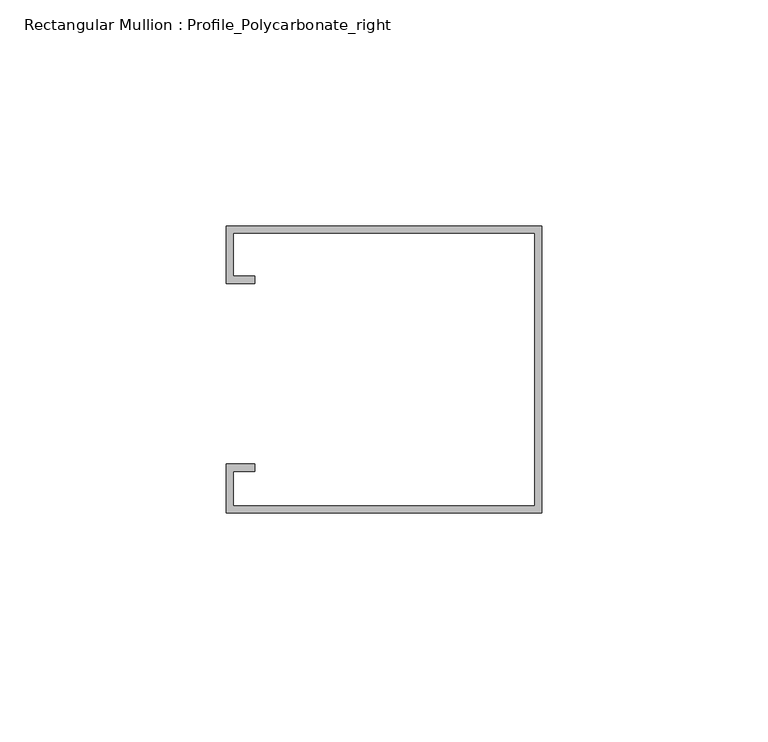
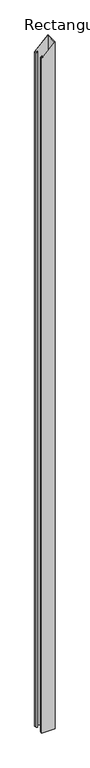
"""IFC4 building model written with IfcOpenShell, lengths in millimetres: member geometry, Rectangular Mullion : Profile_Polycarbonate_right."""

import ifcopenshell
import ifcopenshell.guid

model = None  # the IFC model being written
_history = None  # IfcOwnerHistory: only IFC2X3 demands one
_inside = {}  # id of a spatial element -> (the spatial element, [elements in it])
_under = {}  # id of a project, library or spatial element -> (it, [spatial elements below it])
_declared = {}  # id of a project -> (the project, [libraries it declares])
_typed = {}  # id of a type object -> (the type object, [elements of that type])
_made_of = {}  # id of a material, layer set ... -> (it, [elements and type objects made of it])


def new_model(schema):
    """Start an empty IFC model of exactly this schema.

    Asked for "IFC4X3", IfcOpenShell would pick the latest addendum, in which some entities
    have other attributes; the version numbers below select the first issue.
    IFC2X3 requires an IfcOwnerHistory on every rooted entity: one is made here for all.
    """
    global model, _history
    if schema == "IFC4X3":
        model = ifcopenshell.file(schema_version=(4, 3, 0, 0))
    else:
        model = ifcopenshell.file(schema=schema)
    _inside.clear()
    _under.clear()
    _declared.clear()
    _typed.clear()
    _made_of.clear()
    _history = None
    if model.schema == "IFC2X3":
        org = make("IfcOrganization", Name="unknown")
        user = make(
            "IfcPersonAndOrganization",
            ThePerson=make("IfcPerson", FamilyName="unknown"),
            TheOrganization=org,
        )
        app = make(
            "IfcApplication",
            ApplicationDeveloper=org,
            Version="unknown",
            ApplicationFullName="unknown",
            ApplicationIdentifier="unknown",
        )
        _history = make(
            "IfcOwnerHistory",
            OwningUser=user,
            OwningApplication=app,
            ChangeAction="ADDED",
            CreationDate=0,
        )
    return model


def make(cls, **values):
    """One entity of the class cls with the attributes given. An attribute that is None is left unset."""
    return model.create_entity(
        cls, **{name: value for name, value in values.items() if value is not None}
    )


def rooted(cls, **values):
    """An entity with a GlobalId (a new one), such as an element, a storey or a relation."""
    return make(cls, GlobalId=ifcopenshell.guid.new(), OwnerHistory=_history, **values)


def si_unit(unit_type, name, prefix=None):
    """IfcSIUnit, for example si_unit("LENGTHUNIT", "METRE", prefix="MILLI")."""
    return make("IfcSIUnit", UnitType=unit_type, Prefix=prefix, Name=name)


def assignment(units):
    """IfcUnitAssignment: the units of a project."""
    return None if units is None else make("IfcUnitAssignment", Units=units)


def point(xyz):
    """IfcCartesianPoint."""
    return None if xyz is None else make("IfcCartesianPoint", Coordinates=xyz)


def direction(xyz):
    """IfcDirection."""
    return None if xyz is None else make("IfcDirection", DirectionRatios=xyz)


def frame(location, z_axis=None, x_axis=None):
    """IfcAxis2Placement3D, a coordinate frame: its origin and axes. An axis left out is left unset."""
    return make(
        "IfcAxis2Placement3D",
        Location=point(location),
        Axis=direction(z_axis),
        RefDirection=direction(x_axis),
    )


def origin():
    """The frame at (0, 0, 0) with its axes left unset."""
    return frame((0.0, 0.0, 0.0))


def place(relative_to, where):
    """IfcLocalPlacement: puts the frame where relative to a parent placement (None: the world)."""
    return make(
        "IfcLocalPlacement", PlacementRelTo=relative_to, RelativePlacement=where
    )


def context(
    kind, dimensions, precision=None, world=None, true_north=None, identifier=None
):
    """IfcGeometricRepresentationContext, for example the 3D "Model" context."""
    return make(
        "IfcGeometricRepresentationContext",
        ContextIdentifier=identifier,
        ContextType=kind,
        CoordinateSpaceDimension=dimensions,
        Precision=precision,
        WorldCoordinateSystem=world,
        TrueNorth=true_north,
    )


def project(units=None, contexts=None):
    """IfcProject with its units and contexts."""
    return rooted(
        "IfcProject",
        Name="project",
        RepresentationContexts=contexts,
        UnitsInContext=assignment(units),
    )


def spatial(cls, under=None, at=None, **own):
    """A site, building, storey or space (cls), placed at a placement, below another one or the project."""
    s = rooted(cls, ObjectPlacement=at, **own)
    if under is not None:
        _under.setdefault(under.id(), (under, []))[1].append(s)
    return s


def faces_of(points, faces, orient=None, outer=None):
    """IfcFace entities. A face is a list of loops; a loop is a list of indices into points, from 0.

    orient and outer hold one flag for each loop. By default every Orientation is true, the
    first loop of a face is its IfcFaceOuterBound and the others are IfcFaceBound.
    """
    made = []
    for i, loops in enumerate(faces):
        bounds = []
        for j, loop in enumerate(loops):
            is_outer = j == 0 if outer is None else outer[i][j]
            bounds.append(
                make(
                    "IfcFaceOuterBound" if is_outer else "IfcFaceBound",
                    Bound=make("IfcPolyLoop", Polygon=[points[k] for k in loop]),
                    Orientation=True if orient is None else orient[i][j],
                )
            )
        made.append(make("IfcFace", Bounds=bounds))
    return made


def faceted_brep(points, faces, orient=None, outer=None, voids=None):
    """IfcFacetedBrep: a solid bounded by flat faces; with voids (closed shells), ...WithVoids."""
    shared = [point(p) for p in points]
    hull = make("IfcClosedShell", CfsFaces=faces_of(shared, faces, orient, outer))
    if voids is None:
        return make("IfcFacetedBrep", Outer=hull)
    return make(
        "IfcFacetedBrepWithVoids",
        Outer=hull,
        Voids=[
            make(cls, CfsFaces=faces_of(shared, fs, o, b)) for cls, fs, o, b in voids
        ],
    )


def shape(context_of_items, identifier, shape_type, items):
    """IfcShapeRepresentation: the items that make up one representation, for example the "Body"."""
    return make(
        "IfcShapeRepresentation",
        ContextOfItems=context_of_items,
        RepresentationIdentifier=identifier,
        RepresentationType=shape_type,
        Items=items,
    )


def source(mapping_origin, context_of_items, identifier, shape_type, items):
    """IfcRepresentationMap: a shape defined once, which mapped items show again and again."""
    return make(
        "IfcRepresentationMap",
        MappingOrigin=mapping_origin,
        MappedRepresentation=shape(context_of_items, identifier, shape_type, items),
    )


def transform(
    local_origin,
    x_axis=None,
    y_axis=None,
    z_axis=None,
    scale=None,
    scale2=None,
    scale3=None,
    uniform=True,
):
    """IfcCartesianTransformationOperator3D, or its non-uniform kind. x_axis, y_axis, z_axis: its Axis1, 2, 3."""
    if uniform:
        return make(
            "IfcCartesianTransformationOperator3D",
            Axis1=direction(x_axis),
            Axis2=direction(y_axis),
            LocalOrigin=point(local_origin),
            Scale=scale,
            Axis3=direction(z_axis),
        )
    return make(
        "IfcCartesianTransformationOperator3DnonUniform",
        Axis1=direction(x_axis),
        Axis2=direction(y_axis),
        LocalOrigin=point(local_origin),
        Scale=scale,
        Axis3=direction(z_axis),
        Scale2=scale2,
        Scale3=scale3,
    )


def mapped(mapping_source, mapping_target):
    """IfcMappedItem: shows the shape of a source again, moved by a transform."""
    return make(
        "IfcMappedItem", MappingSource=mapping_source, MappingTarget=mapping_target
    )


def made_of(thing, what):
    """Note that an element or type object is made of a material, layer set ...; save() writes the relation."""
    if what is not None:
        _made_of.setdefault(what.id(), (what, []))[1].append(thing)
    return thing


def element(
    cls,
    number,
    at=None,
    inside=None,
    cuts=None,
    type_object=None,
    material=None,
    context=None,
    identifier="Body",
    shape_type=None,
    held_by="IfcProductDefinitionShape",
    body=None,
    shapes=None,
    **own,
):
    """One element of the class cls, such as IfcWall. Its Tag is "e" and its number.

    at: its placement. inside: the storey or other place that contains it. cuts: it is an
    opening in that element (IfcRelVoidsElement). A single representation is given by context,
    identifier, shape_type and body (its items); several are given by shapes. held_by: the class
    of the entity that holds the representations. save() writes the other relations.
    """
    e = rooted(cls, Tag="e%d" % number, ObjectPlacement=at, **own)
    if body is not None:
        shapes = [shape(context, identifier, shape_type, body)]
    if shapes is not None:
        e.Representation = make(held_by, Representations=shapes)
    if inside is not None:
        _inside.setdefault(inside.id(), (inside, []))[1].append(e)
    if cuts is not None:
        rooted(
            "IfcRelVoidsElement", RelatingBuildingElement=cuts, RelatedOpeningElement=e
        )
    if type_object is not None:
        _typed.setdefault(type_object.id(), (type_object, []))[1].append(e)
    return made_of(e, material)


def aggregate(whole, parts):
    """IfcRelAggregates: a whole, such as a stair, and the parts it consists of."""
    return rooted("IfcRelAggregates", RelatingObject=whole, RelatedObjects=parts)


def save(model, path):
    """Write the relations noted so far, then the file.

    IfcRelAggregates (storeys below a building ...), IfcRelContainedInSpatialStructure (elements
    in a storey), IfcRelDefinesByType, IfcRelAssociatesMaterial and IfcRelDeclares: one each for
    every whole, place, type object, material and project.
    """
    for whole, parts in _under.values():
        aggregate(whole, parts)
    for where, things in _inside.values():
        rooted(
            "IfcRelContainedInSpatialStructure",
            RelatedElements=things,
            RelatingStructure=where,
        )
    for kind, things in _typed.values():
        rooted("IfcRelDefinesByType", RelatedObjects=things, RelatingType=kind)
    for what, things in _made_of.values():
        rooted("IfcRelAssociatesMaterial", RelatedObjects=things, RelatingMaterial=what)
    for by, libraries in _declared.values():
        rooted("IfcRelDeclares", RelatingContext=by, RelatedDefinitions=libraries)
    model.write(path)


def rectangular_mullion_profile_polycarbonate_right_e104eb16(model_context):
    return source(origin(), model_context, "Body", "Brep", [
        faceted_brep([(0.0, 32.7, -3762.4574128), (0.0, -30.8, -3762.4574128), (-69.85, -30.8, -3762.4574128), (-69.85, -20.0, -3762.4574128), (-63.5, -20.0, -3762.4574128), (-63.5, -21.5875, -3762.4574128), (-68.2625, -21.5875, -3762.4574128), (-68.2625, -29.2125, -3762.4574128), (-1.5875, -29.2125, -3762.4574128), (-1.5875, 31.1125, -3762.4574128), (-68.2625, 31.1125, -3762.4574128), (-68.2625, 21.5875, -3762.4574128), (-63.5, 21.5875, -3762.4574128), (-63.5, 20.0, -3762.4574128), (-69.85, 20.0, -3762.4574128), (-69.85, 32.7, -3762.4574128), (-69.85, 32.7, -67.0001907), (0.0, 32.7, 0.0), (-69.85, 20.0, -67.0001907), (-63.5, 20.0, -60.9092643), (-63.5, 21.5875, -60.9092643), (-68.2625, 21.5875, -65.4774591), (-68.2625, 31.1125, -65.4774591), (-1.5875, 31.1125, -1.5227316), (-1.5875, -29.2125, -1.5227316), (-68.2625, -29.2125, -65.4774591), (-68.2625, -21.5875, -65.4774591), (-63.5, -21.5875, -60.9092643), (-63.5, -20.0, -60.9092643), (-69.85, -20.0, -67.0001907), (-69.85, -30.8, -67.0001907), (0.0, -30.8, 0.0)], [[[0, 1, 2, 3, 4, 5, 6, 7, 8, 9, 10, 11, 12, 13, 14, 15]], [[16, 17, 0, 15]], [[18, 16, 15, 14]], [[19, 18, 14, 13]], [[20, 19, 13, 12]], [[21, 20, 12, 11]], [[22, 21, 11, 10]], [[23, 22, 10, 9]], [[24, 23, 9, 8]], [[25, 24, 8, 7]], [[26, 25, 7, 6]], [[27, 26, 6, 5]], [[28, 27, 5, 4]], [[29, 28, 4, 3]], [[30, 29, 3, 2]], [[31, 30, 2, 1]], [[17, 31, 1, 0]], [[17, 16, 18, 19, 20, 21, 22, 23, 24, 25, 26, 27, 28, 29, 30, 31]]]),
    ])


if __name__ == "__main__":
    model = new_model("IFC4")
    model_context = context("Model", 3, world=origin())
    ifc_project = project(units=[si_unit("LENGTHUNIT", "METRE", prefix="MILLI")], contexts=[model_context])
    site = spatial("IfcSite", under=ifc_project)
    building = spatial("IfcBuilding", under=site)
    placement = place(None, origin())
    rectangular_mullion_profile_polycarbonate_right_shape = rectangular_mullion_profile_polycarbonate_right_e104eb16(model_context)
    element("IfcMember", 1, ObjectType="Rectangular Mullion : Profile_Polycarbonate_right", at=placement, inside=building, context=model_context, shape_type="MappedRepresentation", body=[
        mapped(rectangular_mullion_profile_polycarbonate_right_shape, transform((0.0, 0.0, 0.0), x_axis=(1.0, 0.0, 0.0), y_axis=(0.0, 1.0, 0.0), z_axis=(0.0, 0.0, 1.0))),
    ])
    save(model, "model.ifc")

# Revit data of these elements
# Type "Rectangular Mullion : Profile_Polycarbonate_right"
#   built-in parameter 1007322 = 0.208333 (stored number, unit not read)
#   built-in parameter 1007321 = 0 (stored number, unit not read)
#   built-in parameter 1007320 = 0.00520833 (stored number, unit not read)
